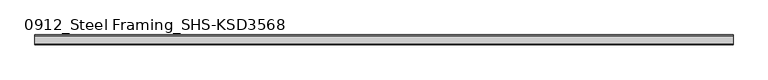
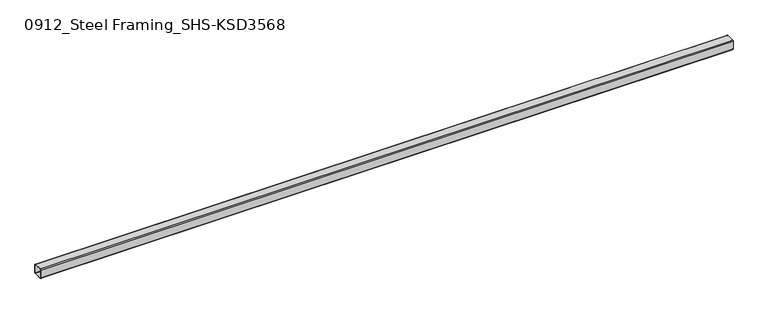
"""IFC4 building model written with IfcOpenShell, lengths in millimetres: beam geometry, 0912_Steel Framing_SHS-KSD3568 : H_SB_ASB_SHS-150x150x6."""

from ifc_helpers import new_model, si_unit, point, frame, frame_2d, origin, place, context, project, spatial, polyline, circle_curve, trimmed, segment, composite_curve, outline, extrude, source, transform, mapped, element, save


def beam_0912_steel_framing_shs_ksd3568_f6c9650c(model_context):
    return source(origin(), model_context, "Body", "SweptSolid", [
        extrude(outline(composite_curve([segment(polyline([(75.0, 63.0), (75.0, -63.0)]), True, "CONTINUOUS"), segment(trimmed(circle_curve(frame_2d((63.0, -63.0)), 12.0), [point((75.0, -63.0))], [point((63.0, -75.0))], False, "CARTESIAN"), True, "CONTINUOUS"), segment(polyline([(63.0, -75.0), (-63.0, -75.0)]), True, "CONTINUOUS"), segment(trimmed(circle_curve(frame_2d((-63.0, -63.0)), 12.0), [point((-63.0, -75.0))], [point((-75.0, -63.0))], False, "CARTESIAN"), True, "CONTINUOUS"), segment(polyline([(-75.0, -63.0), (-75.0, 63.0)]), True, "CONTINUOUS"), segment(trimmed(circle_curve(frame_2d((-63.0, 63.0)), 12.0), [point((-75.0, 63.0))], [point((-63.0, 75.0))], False, "CARTESIAN"), True, "CONTINUOUS"), segment(polyline([(-63.0, 75.0), (63.0, 75.0)]), True, "CONTINUOUS"), segment(trimmed(circle_curve(frame_2d((63.0, 63.0)), 12.0), [point((63.0, 75.0))], [point((75.0, 63.0))], False, "CARTESIAN"), True, "CONTINUOUS")], self_intersect=False), holes=[composite_curve([segment(trimmed(circle_curve(frame_2d((-63.0, 63.0)), 6.0), [point((-63.0, 69.0))], [point((-69.0, 63.0))], True, "CARTESIAN"), True, "CONTINUOUS"), segment(polyline([(-69.0, 63.0), (-69.0, -63.0)]), True, "CONTINUOUS"), segment(trimmed(circle_curve(frame_2d((-63.0, -63.0)), 6.0), [point((-69.0, -63.0))], [point((-63.0, -69.0))], True, "CARTESIAN"), True, "CONTINUOUS"), segment(polyline([(-63.0, -69.0), (63.0, -69.0)]), True, "CONTINUOUS"), segment(trimmed(circle_curve(frame_2d((63.0, -63.0)), 6.0), [point((63.0, -69.0))], [point((69.0, -63.0))], True, "CARTESIAN"), True, "CONTINUOUS"), segment(polyline([(69.0, -63.0), (69.0, 63.0)]), True, "CONTINUOUS"), segment(trimmed(circle_curve(frame_2d((63.0, 63.0)), 6.0), [point((69.0, 63.0))], [point((63.0, 69.0))], True, "CARTESIAN"), True, "CONTINUOUS"), segment(polyline([(63.0, 69.0), (-63.0, 69.0)]), True, "CONTINUOUS")], self_intersect=False)]), frame((-5290.0, 0.0, 0.0), z_axis=(1.0, 0.0, 0.0), x_axis=(0.0, 1.0, 0.0)), (0.0, 0.0, 1.0), 10580.0),
    ])


if __name__ == "__main__":
    model = new_model("IFC4")
    model_context = context("Model", 3, world=origin())
    ifc_project = project(units=[si_unit("LENGTHUNIT", "METRE", prefix="MILLI")], contexts=[model_context])
    site = spatial("IfcSite", under=ifc_project)
    building = spatial("IfcBuilding", under=site)
    placement = place(None, origin())
    beam_0912_steel_framing_shs_ksd3568_shape = beam_0912_steel_framing_shs_ksd3568_f6c9650c(model_context)
    element("IfcBeam", 1, ObjectType="0912_Steel Framing_SHS-KSD3568 : H_SB_ASB_SHS-150x150x6", at=placement, inside=building, context=model_context, shape_type="MappedRepresentation", body=[
        mapped(beam_0912_steel_framing_shs_ksd3568_shape, transform((0.0, 0.0, 0.0), x_axis=(1.0, 0.0, 0.0), y_axis=(0.0, 1.0, 0.0), z_axis=(0.0, 0.0, 1.0))),
    ])
    save(model, "model.ifc")

# Revit data of these elements
# Type "0912_Steel Framing_SHS-KSD3568 : H_SB_ASB_SHS-150x150x6"
#   H_WM Code_1 = "S01AA002-00001 | Main Steel Structure Fabrication Work | Shelter/Building | Medium Steel - Standard (90KG/M>Weight≥30KG/M) | Material: (   )"
#   H_WM Code_2 = "S03AA028-00001 | Main Steel Structure Erection Work | Shelter/Building | Medium Steel (90KG/M>Weight≥30KG/M) | Material: (   )"
#   H_WM Code_3 = "S01AA010-00001 | Main Steel Structure Fabrication Work | Shelter/Building | Steel Painting/Coating | for Non-Fireproofed Steel Surface, Surface Preparation, Primer, Second & Final Coat | Material: (   )"
#   H_Q'ty Cal Type Tag = "SB-Q2"
#   Perimeter = 0.60 m²/m
#   Nominal Weight = 26.40 kgf/m
#   Length [instance default] = 1.0000 m
#   b = 0.1500 m
#   h = 0.1500 m
#   tr = 0.0120 m
#   t = 0.0060 m
#   A = 28.36 m²
#   Structural Material [instance default] = Steel, 45-345
# Element 1 (IfcBeam, "0912_Steel Framing_SHS-KSD3568 : H_SB_ASB_SHS-150x150x6")
#   Structural Material = none
# Materials
#   "Steel, 45-345": class "Metal", colour RGB 189 187 185, transparency 0, Description = "Steel 345 MPa", Cost = 0
